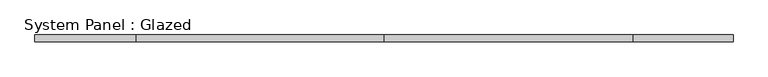
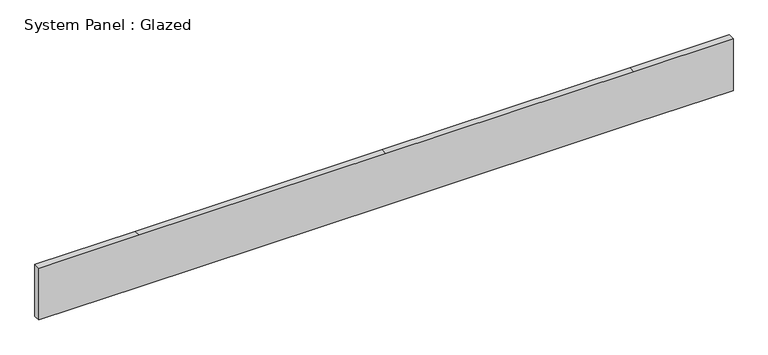
"""IFC4 building model written with IfcOpenShell, lengths in millimetres: plate geometry, System Panel : Glazed."""

from ifc_helpers import new_model, si_unit, frame, origin, place, context, project, spatial, polyline, outline, extrude, source, transform, mapped, element, save


def system_panel_glazed_1a787650(model_context):
    return source(origin(), model_context, "Body", "SweptSolid", [
        extrude(outline(polyline([(0.0, -1328.0571429), (0.0, -943.4285714), (0.0, 0.0), (0.0, 948.8714286), (0.0, 1328.0571429), (209.55, 1328.0571429), (209.55, 948.8714286), (209.55, 0.0), (209.55, -943.4285714), (209.55, -1328.0571429), (0.0, -1328.0571429)])), frame((0.0, 19.05, 0.0), z_axis=(0.0, 1.0, 0.0), x_axis=(0.0, 0.0, 1.0)), (0.0, 0.0, 1.0), 25.4),
    ])


if __name__ == "__main__":
    model = new_model("IFC4")
    model_context = context("Model", 3, world=origin())
    ifc_project = project(units=[si_unit("LENGTHUNIT", "METRE", prefix="MILLI")], contexts=[model_context])
    site = spatial("IfcSite", under=ifc_project)
    building = spatial("IfcBuilding", under=site)
    placement = place(None, origin())
    system_panel_glazed_shape = system_panel_glazed_1a787650(model_context)
    element("IfcPlate", 1, ObjectType="System Panel : Glazed", at=placement, inside=building, context=model_context, shape_type="MappedRepresentation", body=[
        mapped(system_panel_glazed_shape, transform((0.0, 0.0, 0.0), x_axis=(1.0, 0.0, 0.0), y_axis=(0.0, 1.0, 0.0), z_axis=(0.0, 0.0, 1.0))),
    ])
    save(model, "model.ifc")

# Revit data of these elements
# Element 1 (IfcPlate, "System Panel : Glazed")
#   Materials on its faces: "Glass"
# Materials
#   "Glass": class "Glass", colour RGB 0 128 192, transparency 0.75
